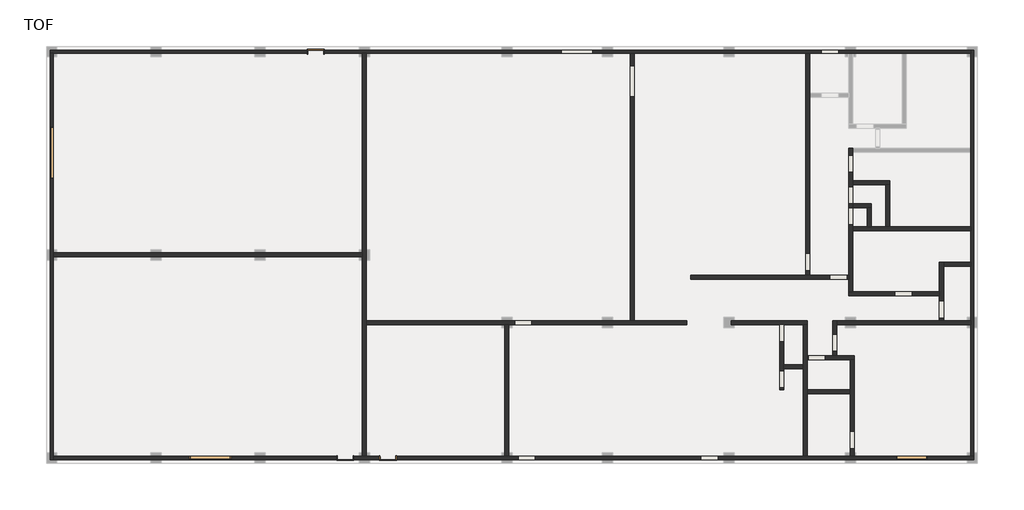
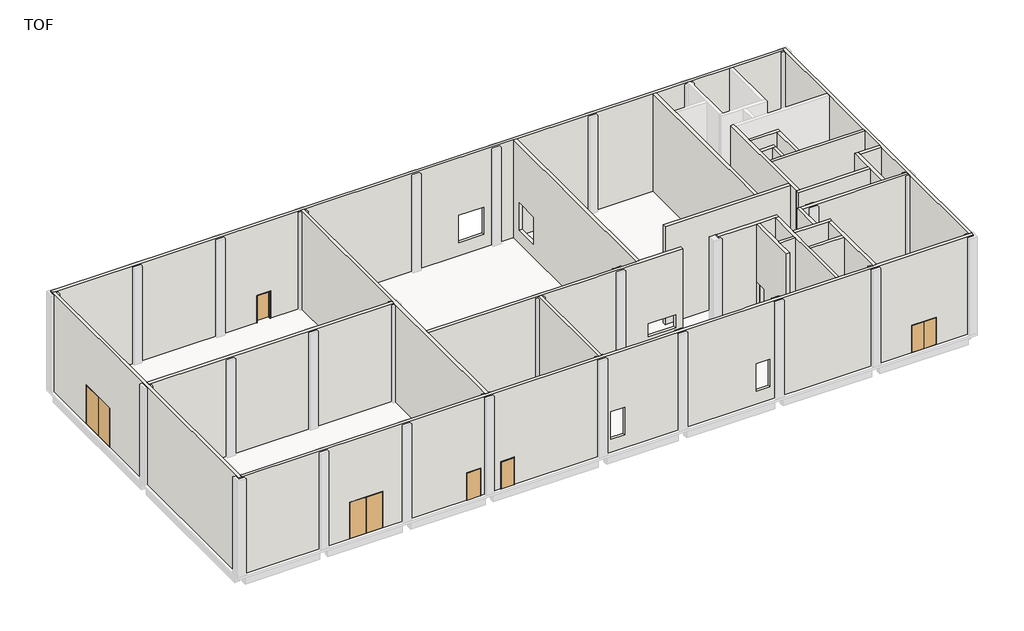
# One storey, part 1 of 2: 29 walls, 6 doors.
# Revit data of these elements (continued)
# Project information
#   H_Seismic Condition = "A as per ASCE 7-10"
#   H_Soil Condition = "C as per ASCE 7-10"
#   H_Basic Wind Speed = "58.3m/s ASCE7-10"
#   Building Name = "Sulfur Loading Control Building"
#   H_DS Project Code = "FAASA2302"
#   H_Project Abbreviation = "SACE2"
#   H_Project Division = "화공"
#   H_Project Finish = "2027-03-05"
#   H_Project Location = "Jafurah, Saudi Arabia"
#   H_Project Start = "2024-01-03"
#   H_Project Type = "EPC"
#   H_Smart Code = "FAASA2302"
#   Project Issue Date = "Issue Date"
#   Project Status = "Project Status"
#   Client Name = "Owner"
#   Project Address = "Enter address here"
#   Project Name = "Japurah2"
#   Project Number = "0001"
# Grids (mm)
#   "Y2": line (-3860.098, 12199.521) -> (22160.842, 12199.521)
#   "X1": line (0, 29277.337) -> (0, -4496.638)
#   "X2": line (6000, 29277.337) -> (6000, -4496.638)
#   "Y1": line (-3860.098, 23899.521) -> (59043.988, 23899.521)
#   "Y3": line (23626.352, 8299.521) -> (59043.988, 8299.521)
#   "Y4": line (-3860.098, 499.521) -> (59043.988, 499.521)
#   "X3": line (12000, 29277.337) -> (12000, -4496.638)
#   "X4": line (18000, 29277.337) -> (18000, -4496.638)
#   "X5": line (26200, 29277.337) -> (26200, -4496.638)
#   "X6": line (32000, 29277.337) -> (32000, -4496.638)
#   "X7": line (39000, 29277.337) -> (39000, -4496.638)
#   "X8": line (46000, 29277.337) -> (46000, -4496.638)
#   "X9": line (53000, 29277.337) -> (53000, -4496.638)
# Type "Double Door_Steel : H_DR_AR_B12_Double Door_Steel_W2000xH2100"
#   Type Mark = ""
#   프레임 = ""
#   철물 = ""
#   유리/마감 = ""
#   위치/개소 = ""
#   부호 = "1/SD"
#   문번호 = ""
#   문기호 = "SD"
#   Analytic Construction = "<None>"
#   Height = 2100 mm
#   Width = 1800 mm
#   Define Thermal Properties by = 1
#   문 틀 = none
#   문 = none
#   Function = (empty or 0)
#   Assembly Code = ""
#   Wall Closure = (empty or 0)
# Type "Double Door_Steel : H_DR_AR_B12_Double Door_Steel_W2400xH2800"
#   Type Mark = "429"
#   프레임 = ""
#   철물 = ""
#   유리/마감 = ""
#   위치/개소 = ""
#   부호 = "1/SD"
#   문번호 = ""
#   문기호 = "SD"
#   Analytic Construction = "<None>"
#   Height = 2800 mm
#   Width = 2400 mm
#   Define Thermal Properties by = 1
#   문 틀 = none
#   문 = none
#   Function = (empty or 0)
#   Assembly Code = ""
#   Wall Closure = (empty or 0)
# Type "Double Door_Steel : H_DR_AR_B12_Double Door_Steel_W3000xH3000"
#   Type Mark = "430"
#   프레임 = ""
#   철물 = ""
#   유리/마감 = ""
#   위치/개소 = ""
#   부호 = "1/SD"
#   문번호 = ""
#   문기호 = "SD"
#   Analytic Construction = "<None>"
#   Height = 3000 mm
#   Width = 3000 mm
#   Define Thermal Properties by = 1
#   문 틀 = none
#   문 = none
#   Function = (empty or 0)
#   Assembly Code = ""
#   Wall Closure = (empty or 0)
# Type "Single Door_Steel : H_DR_AR_B12_Single Door_Steel_W1000xH2100"
#   Type Mark = "SD"
#   Analytic Construction = "<None>"
#   프레임 투영 외부. = 25 mm
#   프레임 투영 내부. = 25 mm
#   프레임 폭 = 75 mm
#   Height = 2100 mm
#   Width = 1000 mm
#   Define Thermal Properties by = 1
#   문 패널 = none
#   문 프레임 = none
#   Function = (empty or 0)
#   Wall Closure = (empty or 0)
# Type "H_WA_AR_B02_Ext Wall_RC T200"
#   Type Comments = ""
#   Layers, outside or top first: 0 mm no material (function 100); 0 mm no material (function 100); 200 mm no material (function 1); 0 mm no material (function 100); 0 mm no material (function 100); 0 mm no material (function 100)
# Type "H_WA_AR_B02_Int Wall_Block T200"
#   Type Comments = ""
#   Layers, outside or top first: 0 mm no material (function 100); 12 mm no material (function 2); 200 mm no material (function 1); 12 mm no material (function 2); 10 mm no material (function 5)
# Element 1 (IfcDoor, "Double Door_Steel : H_DR_AR_B12_Double Door_Steel_W2000xH2100")
#   H_Door Style Name = "Steel Door_Double"
#   H_Door_Frame = "Steel"
#   H_Door_Leaf = "Steel"
#   H_Door_Vision = "N.A"
#   H_Door_Panic = "N.A"
#   H_Door_Style Remark = ""
#   H_Door_Fire Rating = "NA/0.5/1.0\n/1.5/2.0"
#   H_Door Style No = DD11
#   Phase Created = New Construction
# Element 2 (IfcDoor, "Double Door_Steel : H_DR_AR_B12_Double Door_Steel_W2400xH2800")
#   H_Door Style Name = "Steel Door_Double"
#   H_Door_Frame = "Steel"
#   H_Door_Leaf = "Steel"
#   H_Door_Vision = "N.A"
#   H_Door_Panic = "N.A"
#   H_Door_Style Remark = ""
#   H_Door_Fire Rating = "NA/0.5/1.0\n/1.5/2.0"
#   H_Door Style No = DD11
#   Phase Created = New Construction
# Element 3 (IfcDoor, "Double Door_Steel : H_DR_AR_B12_Double Door_Steel_W3000xH3000")
#   H_Door Style Name = "Steel Door_Double"
#   H_Door_Frame = "Steel"
#   H_Door_Leaf = "Steel"
#   H_Door_Vision = "N.A"
#   H_Door_Panic = "N.A"
#   H_Door_Style Remark = ""
#   H_Door_Fire Rating = "NA/0.5/1.0\n/1.5/2.0"
#   H_Door Style No = DD11
#   Phase Created = New Construction
# Elements 4, 5, 6 (IfcDoor, "Single Door_Steel : H_DR_AR_B12_Single Door_Steel_W1000xH2100")
#   H_Door Style Name = "Steel Door_Single"
#   H_Door_Frame = "Steel"
#   H_Door_Leaf = "Steel"
#   H_Door_Vision = "N.A"
#   H_Door_Panic = "N.A"
#   H_Door_Style Remark = "Steel Door w/ Steel Frame"
#   H_Door_Fire Rating = "NA/0.5/1.0\n/1.5/2.0"
#   H_Door Style No = SD11
#   Phase Created = New Construction
# Elements 7, 8, 9, 10 (IfcWall, "H_WA_AR_B02_Ext Wall_RC T200")
#   H_Wall Style Name = "Gypsum Board Wall+Mineral Wool Insulation w/ Air Space+Concrete Wall+Acrylic Emulsion Paint on Fair Faced Concrete"
#   H_Wall-Base Material-1 = "1-Layer Gypsum Board"
#   H_Wall-Base Material-2 = "Mineral Wool (Rock Wool)+Air Space"
#   H_Wall_Finish-In = "Acrylic Emulsion Paint"
#   H_Wall_Base Material-3 = "Concrete Wall"
#   H_Wall_Finish-Ex = "Acrylic Emulsion Paint on Fair Faced Concrete"
#   H_Wall_Style Remark = "WM : Plasterboard Dry Liner System (A04AS176-00001~00009)\n        - Gypsum Board + Insulation\n        (Gypsumboard THK=9.5 & 12.5 & 16 mm)"
#   Top Offset = 0 mm
#   Base Offset = 0 mm
#   wall height = 7500 mm
#   H_Wall Style No = EW11
#   Phase Created = New Construction
#   Base Constraint = TOF
#   Top Constraint = TOC
#   Materials on its faces: "Default Wall"
# Elements 11, 12, 13, 14, 15, 16, 17, 18, 19, 20, 21, 22, 23, 24, 25, 26, 27, 28, 29, 30, 31, 32, 33, 34, 35 (IfcWall, "H_WA_AR_B02_Int Wall_Block T200")
#   H_Wall Style Name = "Block Wall"
#   H_Wall-Base Material-1 = "Concrete Block"
#   H_Wall-Base Material-2 = ""
#   H_Wall_Finish-In = "Acrylic Emulsion Paint on Cement Plaster"
#   H_Wall_Base Material-3 = ""
#   H_Wall_Finish-Ex = "Acrylic Emulsion Paint on Cement Plaster"
#   H_Wall_Style Remark = "WM : Reinforced Concrete Block\n     50mm<THK≤100mm / 100mm<THK≤200mm / 200mm<THK"
#   Top Offset = 0 mm
#   Base Offset = 0 mm
#   wall height = 7500 mm
#   H_Wall Style No = IW21
#   Phase Created = New Construction
#   Base Constraint = TOF
#   Top Constraint = TOC
#   Materials on its faces: "Default Wall"
# Materials
#   "Default Wall": class "Miscellaneous", colour RGB 80 80 80, transparency 0
